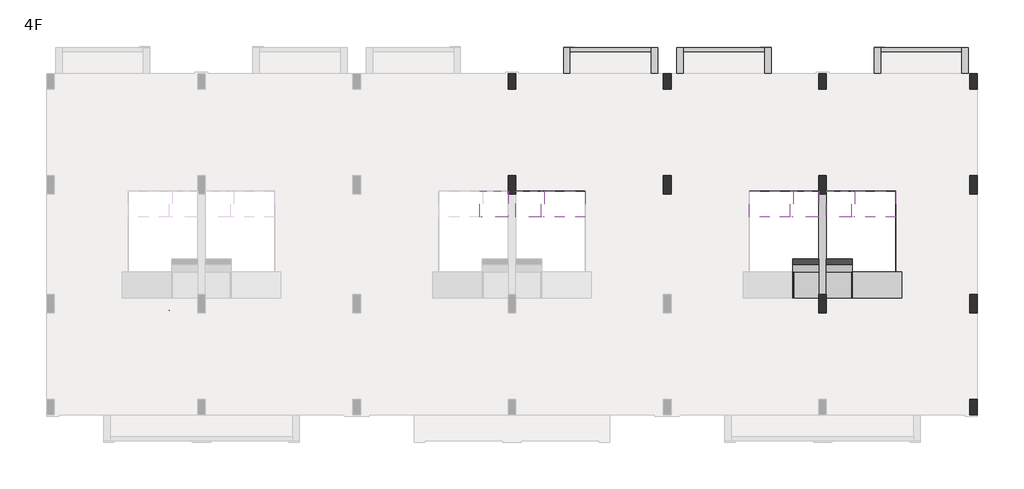
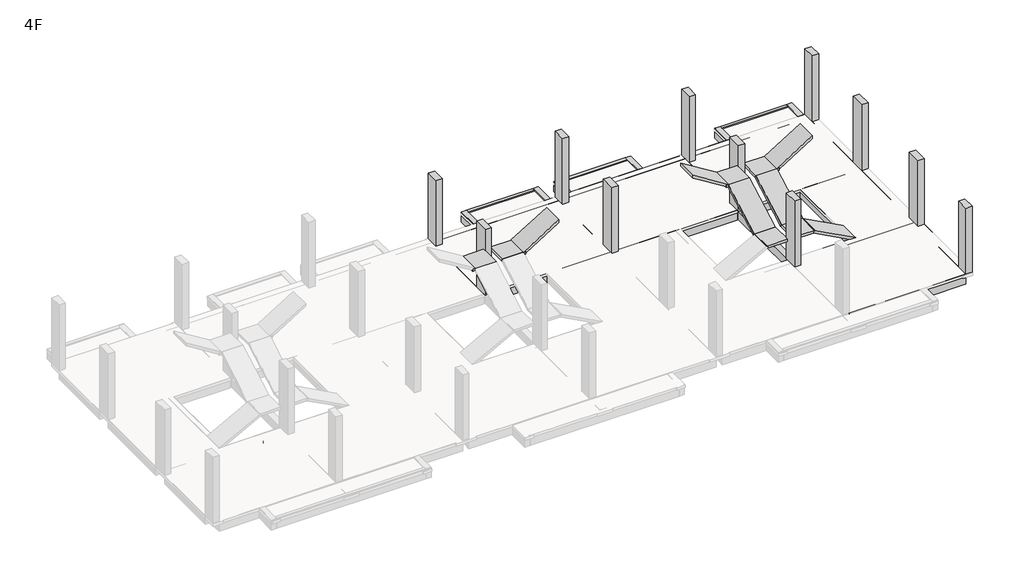
# One storey, part 3 of 3: 37 beams, 11 columns, 1 proxy.
"""IFC4 building model written with IfcOpenShell, lengths in millimetres."""

import ifcopenshell
import ifcopenshell.guid

model = None  # the IFC model being written
_history = None  # IfcOwnerHistory: only IFC2X3 demands one
_inside = {}  # id of a spatial element -> (the spatial element, [elements in it])
_under = {}  # id of a project, library or spatial element -> (it, [spatial elements below it])
_declared = {}  # id of a project -> (the project, [libraries it declares])
_typed = {}  # id of a type object -> (the type object, [elements of that type])
_made_of = {}  # id of a material, layer set ... -> (it, [elements and type objects made of it])


def new_model(schema):
    """Start an empty IFC model of exactly this schema.

    Asked for "IFC4X3", IfcOpenShell would pick the latest addendum, in which some entities
    have other attributes; the version numbers below select the first issue.
    IFC2X3 requires an IfcOwnerHistory on every rooted entity: one is made here for all.
    """
    global model, _history
    if schema == "IFC4X3":
        model = ifcopenshell.file(schema_version=(4, 3, 0, 0))
    else:
        model = ifcopenshell.file(schema=schema)
    _inside.clear()
    _under.clear()
    _declared.clear()
    _typed.clear()
    _made_of.clear()
    _history = None
    if model.schema == "IFC2X3":
        org = make("IfcOrganization", Name="unknown")
        user = make(
            "IfcPersonAndOrganization",
            ThePerson=make("IfcPerson", FamilyName="unknown"),
            TheOrganization=org,
        )
        app = make(
            "IfcApplication",
            ApplicationDeveloper=org,
            Version="unknown",
            ApplicationFullName="unknown",
            ApplicationIdentifier="unknown",
        )
        _history = make(
            "IfcOwnerHistory",
            OwningUser=user,
            OwningApplication=app,
            ChangeAction="ADDED",
            CreationDate=0,
        )
    return model


def make(cls, **values):
    """One entity of the class cls with the attributes given. An attribute that is None is left unset."""
    return model.create_entity(
        cls, **{name: value for name, value in values.items() if value is not None}
    )


def rooted(cls, **values):
    """An entity with a GlobalId (a new one), such as an element, a storey or a relation."""
    return make(cls, GlobalId=ifcopenshell.guid.new(), OwnerHistory=_history, **values)


def si_unit(unit_type, name, prefix=None):
    """IfcSIUnit, for example si_unit("LENGTHUNIT", "METRE", prefix="MILLI")."""
    return make("IfcSIUnit", UnitType=unit_type, Prefix=prefix, Name=name)


def assignment(units):
    """IfcUnitAssignment: the units of a project."""
    return None if units is None else make("IfcUnitAssignment", Units=units)


def point(xyz):
    """IfcCartesianPoint."""
    return None if xyz is None else make("IfcCartesianPoint", Coordinates=xyz)


def direction(xyz):
    """IfcDirection."""
    return None if xyz is None else make("IfcDirection", DirectionRatios=xyz)


def frame(location, z_axis=None, x_axis=None):
    """IfcAxis2Placement3D, a coordinate frame: its origin and axes. An axis left out is left unset."""
    return make(
        "IfcAxis2Placement3D",
        Location=point(location),
        Axis=direction(z_axis),
        RefDirection=direction(x_axis),
    )


def frame_2d(location, x_axis=None):
    """IfcAxis2Placement2D, a coordinate frame in the plane: its origin and x axis."""
    return make(
        "IfcAxis2Placement2D", Location=point(location), RefDirection=direction(x_axis)
    )


def origin():
    """The frame at (0, 0, 0) with its axes left unset."""
    return frame((0.0, 0.0, 0.0))


def origin_with_axes():
    """The frame at (0, 0, 0) with the z axis (0, 0, 1) and the x axis (1, 0, 0) written out."""
    return frame((0.0, 0.0, 0.0), z_axis=(0.0, 0.0, 1.0), x_axis=(1.0, 0.0, 0.0))


def place(relative_to, where):
    """IfcLocalPlacement: puts the frame where relative to a parent placement (None: the world)."""
    return make(
        "IfcLocalPlacement", PlacementRelTo=relative_to, RelativePlacement=where
    )


def context(
    kind, dimensions, precision=None, world=None, true_north=None, identifier=None
):
    """IfcGeometricRepresentationContext, for example the 3D "Model" context."""
    return make(
        "IfcGeometricRepresentationContext",
        ContextIdentifier=identifier,
        ContextType=kind,
        CoordinateSpaceDimension=dimensions,
        Precision=precision,
        WorldCoordinateSystem=world,
        TrueNorth=true_north,
    )


def project(units=None, contexts=None):
    """IfcProject with its units and contexts."""
    return rooted(
        "IfcProject",
        Name="project",
        RepresentationContexts=contexts,
        UnitsInContext=assignment(units),
    )


def spatial(cls, under=None, at=None, **own):
    """A site, building, storey or space (cls), placed at a placement, below another one or the project."""
    s = rooted(cls, ObjectPlacement=at, **own)
    if under is not None:
        _under.setdefault(under.id(), (under, []))[1].append(s)
    return s


def polyline(points):
    """IfcPolyline through the points."""
    return make("IfcPolyline", Points=[point(p) for p in points])


def circle_curve(where, radius):
    """IfcCircle in the frame where."""
    return make("IfcCircle", Position=where, Radius=radius)


def ellipse_curve(where, semi_axis1, semi_axis2):
    """IfcEllipse in the frame where."""
    return make(
        "IfcEllipse", Position=where, SemiAxis1=semi_axis1, SemiAxis2=semi_axis2
    )


def trimmed(basis, trim1, trim2, sense, master):
    """IfcTrimmedCurve: the piece of a basis curve between two trims."""
    return make(
        "IfcTrimmedCurve",
        BasisCurve=basis,
        Trim1=trim1,
        Trim2=trim2,
        SenseAgreement=sense,
        MasterRepresentation=master,
    )


def segment(curve, same_sense, transition):
    """IfcCompositeCurveSegment."""
    return make(
        "IfcCompositeCurveSegment",
        Transition=transition,
        SameSense=same_sense,
        ParentCurve=curve,
    )


def composite_curve(segments, self_intersect=None):
    """IfcCompositeCurve: segments joined end to end."""
    return make("IfcCompositeCurve", Segments=segments, SelfIntersect=self_intersect)


def outline(outer, holes=None, kind="AREA"):
    """IfcArbitraryClosedProfileDef: a profile drawn as a closed curve; with holes, ...WithVoids."""
    if holes is None:
        return make("IfcArbitraryClosedProfileDef", ProfileType=kind, OuterCurve=outer)
    return make(
        "IfcArbitraryProfileDefWithVoids",
        ProfileType=kind,
        OuterCurve=outer,
        InnerCurves=holes,
    )


def extrude(swept, where, along, depth):
    """IfcExtrudedAreaSolid: the profile swept, set in the frame where, extruded along a direction by depth."""
    return make(
        "IfcExtrudedAreaSolid",
        SweptArea=swept,
        Position=where,
        ExtrudedDirection=direction(along),
        Depth=depth,
    )


def faces_of(points, faces, orient=None, outer=None):
    """IfcFace entities. A face is a list of loops; a loop is a list of indices into points, from 0.

    orient and outer hold one flag for each loop. By default every Orientation is true, the
    first loop of a face is its IfcFaceOuterBound and the others are IfcFaceBound.
    """
    made = []
    for i, loops in enumerate(faces):
        bounds = []
        for j, loop in enumerate(loops):
            is_outer = j == 0 if outer is None else outer[i][j]
            bounds.append(
                make(
                    "IfcFaceOuterBound" if is_outer else "IfcFaceBound",
                    Bound=make("IfcPolyLoop", Polygon=[points[k] for k in loop]),
                    Orientation=True if orient is None else orient[i][j],
                )
            )
        made.append(make("IfcFace", Bounds=bounds))
    return made


def faceted_brep(points, faces, orient=None, outer=None, voids=None):
    """IfcFacetedBrep: a solid bounded by flat faces; with voids (closed shells), ...WithVoids."""
    shared = [point(p) for p in points]
    hull = make("IfcClosedShell", CfsFaces=faces_of(shared, faces, orient, outer))
    if voids is None:
        return make("IfcFacetedBrep", Outer=hull)
    return make(
        "IfcFacetedBrepWithVoids",
        Outer=hull,
        Voids=[
            make(cls, CfsFaces=faces_of(shared, fs, o, b)) for cls, fs, o, b in voids
        ],
    )


def shape(context_of_items, identifier, shape_type, items):
    """IfcShapeRepresentation: the items that make up one representation, for example the "Body"."""
    return make(
        "IfcShapeRepresentation",
        ContextOfItems=context_of_items,
        RepresentationIdentifier=identifier,
        RepresentationType=shape_type,
        Items=items,
    )


def source(mapping_origin, context_of_items, identifier, shape_type, items):
    """IfcRepresentationMap: a shape defined once, which mapped items show again and again."""
    return make(
        "IfcRepresentationMap",
        MappingOrigin=mapping_origin,
        MappedRepresentation=shape(context_of_items, identifier, shape_type, items),
    )


def transform(
    local_origin,
    x_axis=None,
    y_axis=None,
    z_axis=None,
    scale=None,
    scale2=None,
    scale3=None,
    uniform=True,
):
    """IfcCartesianTransformationOperator3D, or its non-uniform kind. x_axis, y_axis, z_axis: its Axis1, 2, 3."""
    if uniform:
        return make(
            "IfcCartesianTransformationOperator3D",
            Axis1=direction(x_axis),
            Axis2=direction(y_axis),
            LocalOrigin=point(local_origin),
            Scale=scale,
            Axis3=direction(z_axis),
        )
    return make(
        "IfcCartesianTransformationOperator3DnonUniform",
        Axis1=direction(x_axis),
        Axis2=direction(y_axis),
        LocalOrigin=point(local_origin),
        Scale=scale,
        Axis3=direction(z_axis),
        Scale2=scale2,
        Scale3=scale3,
    )


def mapped(mapping_source, mapping_target):
    """IfcMappedItem: shows the shape of a source again, moved by a transform."""
    return make(
        "IfcMappedItem", MappingSource=mapping_source, MappingTarget=mapping_target
    )


def made_of(thing, what):
    """Note that an element or type object is made of a material, layer set ...; save() writes the relation."""
    if what is not None:
        _made_of.setdefault(what.id(), (what, []))[1].append(thing)
    return thing


def element(
    cls,
    number,
    at=None,
    inside=None,
    cuts=None,
    type_object=None,
    material=None,
    context=None,
    identifier="Body",
    shape_type=None,
    held_by="IfcProductDefinitionShape",
    body=None,
    shapes=None,
    **own,
):
    """One element of the class cls, such as IfcWall. Its Tag is "e" and its number.

    at: its placement. inside: the storey or other place that contains it. cuts: it is an
    opening in that element (IfcRelVoidsElement). A single representation is given by context,
    identifier, shape_type and body (its items); several are given by shapes. held_by: the class
    of the entity that holds the representations. save() writes the other relations.
    """
    e = rooted(cls, Tag="e%d" % number, ObjectPlacement=at, **own)
    if body is not None:
        shapes = [shape(context, identifier, shape_type, body)]
    if shapes is not None:
        e.Representation = make(held_by, Representations=shapes)
    if inside is not None:
        _inside.setdefault(inside.id(), (inside, []))[1].append(e)
    if cuts is not None:
        rooted(
            "IfcRelVoidsElement", RelatingBuildingElement=cuts, RelatedOpeningElement=e
        )
    if type_object is not None:
        _typed.setdefault(type_object.id(), (type_object, []))[1].append(e)
    return made_of(e, material)


def aggregate(whole, parts):
    """IfcRelAggregates: a whole, such as a stair, and the parts it consists of."""
    return rooted("IfcRelAggregates", RelatingObject=whole, RelatedObjects=parts)


def save(model, path):
    """Write the relations noted so far, then the file.

    IfcRelAggregates (storeys below a building ...), IfcRelContainedInSpatialStructure (elements
    in a storey), IfcRelDefinesByType, IfcRelAssociatesMaterial and IfcRelDeclares: one each for
    every whole, place, type object, material and project.
    """
    for whole, parts in _under.values():
        aggregate(whole, parts)
    for where, things in _inside.values():
        rooted(
            "IfcRelContainedInSpatialStructure",
            RelatedElements=things,
            RelatingStructure=where,
        )
    for kind, things in _typed.values():
        rooted("IfcRelDefinesByType", RelatedObjects=things, RelatingType=kind)
    for what, things in _made_of.values():
        rooted("IfcRelAssociatesMaterial", RelatedObjects=things, RelatingMaterial=what)
    for by, libraries in _declared.values():
        rooted("IfcRelDeclares", RelatingContext=by, RelatedDefinitions=libraries)
    model.write(path)


def plane_surface(at):
    """IfcPlane: the flat surface through the origin of the frame at, square to its z axis."""
    return make("IfcPlane", Position=at)


def cylinder_surface(at, radius):
    """IfcCylindricalSurface: all points at the distance radius from the z axis of the frame at."""
    return make("IfcCylindricalSurface", Position=at, Radius=radius)


def revolved_surface(curve, axis_point, axis_direction):
    """IfcSurfaceOfRevolution: the curve turned about the line through axis_point along axis_direction."""
    return make(
        "IfcSurfaceOfRevolution",
        SweptCurve=make("IfcArbitraryOpenProfileDef", ProfileType="CURVE", Curve=curve),
        AxisPosition=make("IfcAxis1Placement", Location=point(axis_point), Axis=direction(axis_direction)),
    )


def advanced_brep(points, edges, surfaces, faces):
    """IfcAdvancedBrep: a solid bounded by faces that lie on surfaces and meet in shared edges.

    An edge is (start, end): straight between two places in points (the first is 0);
    or (start, end, curve); or (start, end, curve, False) where it runs against its curve.
    A face is (place in surfaces, loops), or (place, loops, False) where it looks against
    its surface's normal. A loop lists edges by number (the first is 1), with a minus sign
    where the edge is run from its end to its start. The first loop is the outer one.
    """
    corners = [point(p) for p in points]
    vertices = [make("IfcVertexPoint", VertexGeometry=c) for c in corners]
    made = []
    for start, end, *more in edges:
        made.append(
            make(
                "IfcEdgeCurve",
                EdgeStart=vertices[start],
                EdgeEnd=vertices[end],
                EdgeGeometry=more[0] if more else make("IfcPolyline", Points=[corners[start], corners[end]]),
                SameSense=more[1] if len(more) > 1 else True,
            )
        )
    hull = []
    for where, loops, *sense in faces:
        bounds = []
        for j, loop in enumerate(loops):
            ring = [make("IfcOrientedEdge", EdgeElement=made[abs(k) - 1], Orientation=k > 0) for k in loop]
            bounds.append(
                make(
                    "IfcFaceOuterBound" if j == 0 else "IfcFaceBound",
                    Bound=make("IfcEdgeLoop", EdgeList=ring),
                    Orientation=True,
                )
            )
        hull.append(make("IfcAdvancedFace", Bounds=bounds, FaceSurface=surfaces[where], SameSense=sense[0] if sense else True))
    return make("IfcAdvancedBrep", Outer=make("IfcClosedShell", CfsFaces=hull))


def m_support_metal_circular_m_support_metal_circular_a779fbb7(model_context):
    return source(origin(), model_context, "Body", "SolidModel", [
        advanced_brep(
        [(-6.0, 0.0, 0.0), (6.0, 0.0, 0.0), (-6.0, 0.0, -63.0), (6.0, 0.0, -63.0), (6.0, 12.0, -75.0), (-6.0, 12.0, -75.0), (-6.0, 63.0, -75.0), (6.0, 63.0, -75.0)],
        [
            (0, 1, circle_curve(origin_with_axes(), 6.0)),
            (1, 0, circle_curve(origin_with_axes(), 6.0)),
            (0, 2),
            (2, 3, circle_curve(frame((0.0, 0.0, -63.0), z_axis=(0.0, 0.0, 1.0), x_axis=(1.0, 0.0, 0.0)), 6.0)),
            (3, 1),
            (3, 2, circle_curve(frame((0.0, 0.0, -63.0), z_axis=(0.0, 0.0, 1.0), x_axis=(1.0, 0.0, 0.0)), 6.0)),
            (4, 3, circle_curve(frame((6.0, 12.0, -63.0), z_axis=(-1.0, 0.0, 0.0), x_axis=(0.0, -1.0, 0.0)), 12.0)),
            (2, 5, circle_curve(frame((-6.0, 12.0, -63.0), z_axis=(1.0, 0.0, 0.0), x_axis=(0.0, -1.0, 0.0)), 12.0)),
            (5, 4, circle_curve(frame((0.0, 12.0, -75.0), z_axis=(0.0, -1.0, 0.0), x_axis=(1.0, 0.0, 0.0)), 6.0)),
            (4, 5, circle_curve(frame((0.0, 12.0, -75.0), z_axis=(0.0, -1.0, 0.0), x_axis=(1.0, 0.0, 0.0)), 6.0)),
            (6, 7, circle_curve(frame((0.0, 63.0, -75.0), z_axis=(0.0, 1.0, 0.0), x_axis=(1.0, 0.0, 0.0)), 6.0)),
            (7, 6, circle_curve(frame((0.0, 63.0, -75.0), z_axis=(0.0, 1.0, 0.0), x_axis=(1.0, 0.0, 0.0)), 6.0)),
            (5, 6),
            (7, 4),
        ],
        [
            plane_surface(origin_with_axes()),
            cylinder_surface(origin_with_axes(), 6.0),
            revolved_surface(trimmed(ellipse_curve(frame((0.0, 0.0, -63.0), z_axis=(0.0, 0.0, 1.0), x_axis=(1.0, 0.0, 0.0)), 6.0, 6.0), [point((-6.0, 0.0, -63.0))], [point((6.0, 0.0, -63.0))], True, "CARTESIAN"), (0.0, 12.0, -63.0), (1.0, 0.0, 0.0)),
            revolved_surface(trimmed(ellipse_curve(frame((0.0, 0.0, -63.0), z_axis=(0.0, 0.0, 1.0), x_axis=(1.0, 0.0, 0.0)), 6.0, 6.0), [point((6.0, 0.0, -63.0))], [point((-6.0, 0.0, -63.0))], True, "CARTESIAN"), (0.0, 12.0, -63.0), (1.0, 0.0, 0.0)),
            plane_surface(frame((0.0, 63.0, -75.0), z_axis=(0.0, 1.0, 0.0), x_axis=(1.0, 0.0, 0.0))),
            cylinder_surface(frame((0.0, 12.0, -75.0), z_axis=(0.0, -1.0, 0.0), x_axis=(1.0, 0.0, 0.0)), 6.0),
        ],
        [
            (0, [[1, 2]]),
            (1, [[-1, 3, 4, 5]]),
            (1, [[-2, -5, 6, -3]]),
            (2, [[7, -4, 8, 9]]),
            (3, [[-8, -6, -7, 10]]),
            (4, [[11, 12]]),
            (5, [[-9, 13, -12, 14]]),
            (5, [[-10, -14, -11, -13]]),
        ],
    ),
        extrude(outline(composite_curve([segment(trimmed(circle_curve(frame_2d((-75.0, 0.0)), 25.0), [point((-75.0, -25.0))], [point((-75.0, 25.0))], False, "CARTESIAN"), True, "CONTINUOUS"), segment(trimmed(circle_curve(frame_2d((-75.0, 0.0)), 25.0), [point((-75.0, 25.0))], [point((-75.0, -25.0))], False, "CARTESIAN"), True, "CONTINUOUS")], self_intersect=False)), frame((0.0, 63.0, 0.0), z_axis=(0.0, 1.0, 0.0), x_axis=(0.0, 0.0, 1.0)), (0.0, 0.0, 1.0), 12.0),
    ])


model = new_model("IFC4")

# Units and contexts
model_context = context("Model", 3, world=origin())
ifc_project = project(units=[si_unit("LENGTHUNIT", "METRE", prefix="MILLI")], contexts=[model_context])

# Site, building, storey
site = spatial("IfcSite", under=ifc_project)
building = spatial("IfcBuilding", under=site)
storey = spatial("IfcBuildingStorey", under=building, Name="4F", Elevation=10630.0)

# Beams
placement = place(None, origin())
element("IfcBeam", 1, ObjectType="M_Concrete-Rectangular Beam : 1000x120", at=placement, inside=storey, context=model_context, shape_type="Brep", body=[
    faceted_brep([(16600.0000058, 7550.0000002, 12880.0), (16600.0000058, 8550.0000002, 12880.0), (16600.0000058, 8550.0000002, 12760.0), (16600.0000058, 7550.0000002, 12760.0), (17700.0000058, 8550.0000002, 12760.0), (17700.0000058, 8550.0000002, 12880.0), (17700.0000058, 7550.0000002, 12880.0), (17700.0000058, 7609.0063595, 12775.5095719), (17700.0000058, 7581.5414925, 12760.0), (16700.0000058, 7550.0000002, 12880.0), (16700.0000058, 7581.5414925, 12760.0), (16700.0000058, 7550.0000002, 12760.0), (16700.0000058, 7609.0063595, 12775.5095719)], [[[0, 1, 2, 3]], [[4, 5, 6, 7, 8]], [[1, 0, 9, 6, 5]], [[2, 1, 5, 4]], [[3, 2, 4, 8, 10, 11]], [[0, 3, 11, 9]], [[12, 7, 6, 9]], [[7, 12, 10, 8]], [[12, 9, 11, 10]]]),
])
element("IfcBeam", 2, ObjectType="M_Concrete-Rectangular Beam : 1000x120", at=placement, inside=storey, context=model_context, shape_type="Brep", body=[
    faceted_brep([(19100.0000058, 8550.0000002, 12880.0), (19100.0000058, 7550.0000002, 12880.0), (19100.0000058, 7550.0000002, 12760.0), (19100.0000058, 8550.0000002, 12760.0), (18000.0000058, 8550.0000002, 12880.0), (18000.0000058, 8550.0000002, 12760.0), (18000.0000058, 7581.5414925, 12760.0), (18000.0000058, 7609.0063595, 12775.5095719), (18000.0000058, 7550.0000002, 12880.0), (19000.0000058, 7550.0000002, 12880.0), (19000.0000058, 7550.0000002, 12760.0), (19000.0000058, 7581.5414925, 12760.0), (19000.0000058, 7609.0063595, 12775.5095719)], [[[0, 1, 2, 3]], [[4, 5, 6, 7, 8]], [[1, 0, 4, 8, 9]], [[0, 3, 5, 4]], [[3, 2, 10, 11, 6, 5]], [[2, 1, 9, 10]], [[12, 9, 8, 7]], [[12, 7, 6, 11]], [[9, 12, 11, 10]]]),
])
element("IfcBeam", 3, ObjectType="M_Concrete-Rectangular Beam : 1000x120", at=placement, inside=storey, context=model_context, shape_type="Brep", body=[
    faceted_brep([(18984.2496976, 7549.9999993, 12880.0), (20680.0000464, 7549.9999993, 13930.0), (20680.0000058, 8549.9999993, 13929.9999748), (18984.2496976, 8549.9999993, 12880.0), (20680.0000058, 8549.9999993, 13788.8582241), (19100.0000058, 8549.9999993, 12810.5302519), (19100.0000058, 8549.9999993, 12880.0), (19100.0000058, 7549.9999993, 12810.5302519), (20680.0000058, 7549.9999993, 13788.8582241), (19000.0000058, 7549.9999993, 12880.0), (19100.0000058, 7549.9999993, 12880.0)], [[[0, 1, 2, 3]], [[3, 2, 4, 5, 6]], [[7, 5, 4, 8]], [[1, 0, 9, 10, 7, 8]], [[10, 6, 5, 7]], [[6, 10, 9, 0, 3]], [[2, 1, 8, 4]]]),
])
element("IfcBeam", 4, ObjectType="M_Concrete-Rectangular Beam : 1000x120", at=placement, inside=storey, context=model_context, shape_type="Brep", body=[
    faceted_brep([(28700.0000039, 7550.0000002, 12880.0), (29700.0000039, 7550.0000002, 12880.0), (29700.0000039, 7609.0063595, 12775.5095719), (28700.0000039, 7609.0063595, 12775.5095719), (28700.0000039, 5424.9999998, 11680.0), (28700.0000039, 5484.0063591, 11575.5095719), (29700.0000039, 5484.0063591, 11575.5095719), (29700.0000039, 5424.9999998, 11680.0), (29700.0000039, 5524.9999998, 11598.6589219), (29700.0000039, 7581.5414925, 12760.0), (28700.0000039, 5524.9999998, 11598.6589219), (28700.0000039, 7581.5414925, 12760.0)], [[[0, 1, 2, 3]], [[4, 5, 6, 7]], [[1, 0, 4, 7]], [[2, 1, 7, 6, 8, 9]], [[3, 2, 9, 8, 6, 5, 10, 11]], [[0, 3, 11, 10, 5, 4]]]),
])
element("IfcBeam", 5, ObjectType="M_Concrete-Rectangular Beam : 1000x120", at=placement, inside=storey, context=model_context, shape_type="Brep", body=[
    faceted_brep([(28600.0000039, 7550.0000002, 12880.0), (28600.0000039, 8550.0000002, 12880.0), (28600.0000039, 8550.0000002, 12760.0), (28600.0000039, 7550.0000002, 12760.0), (29700.0000039, 8550.0000002, 12760.0), (29700.0000039, 8550.0000002, 12880.0), (29700.0000039, 7550.0000002, 12880.0), (29700.0000039, 7609.0063595, 12775.5095719), (29700.0000039, 7581.5414925, 12760.0), (28700.0000039, 7550.0000002, 12880.0), (28700.0000039, 7581.5414925, 12760.0), (28700.0000039, 7550.0000002, 12760.0), (28700.0000039, 7609.0063595, 12775.5095719)], [[[0, 1, 2, 3]], [[4, 5, 6, 7, 8]], [[1, 0, 9, 6, 5]], [[2, 1, 5, 4]], [[3, 2, 4, 8, 10, 11]], [[0, 3, 11, 9]], [[12, 7, 6, 9]], [[7, 12, 10, 8]], [[12, 9, 11, 10]]]),
])
element("IfcBeam", 6, ObjectType="M_Concrete-Rectangular Beam : 1000x120", at=placement, inside=storey, context=model_context, shape_type="Brep", body=[
    faceted_brep([(27019.9999632, 7549.9999993, 13930.0), (28715.750312, 7549.9999993, 12880.0), (28715.750312, 8549.9999993, 12880.0), (27019.9999632, 8549.9999993, 13930.0), (28600.0000039, 8549.9999993, 12880.0), (28600.0000039, 8549.9999993, 12810.5302519), (27020.000004, 8549.9999993, 13788.8582239), (28600.0000039, 7549.9999993, 12810.5302519), (27020.000004, 7549.9999993, 13788.8582239), (28600.0000039, 7549.9999993, 12880.0), (28700.0000039, 7549.9999993, 12880.0)], [[[0, 1, 2, 3]], [[3, 2, 4, 5, 6]], [[5, 7, 8, 6]], [[1, 0, 8, 7, 9, 10]], [[4, 9, 7, 5]], [[9, 4, 2, 1, 10]], [[0, 3, 6, 8]]]),
])
element("IfcBeam", 7, ObjectType="M_Concrete-Rectangular Beam : 1000x120", at=placement, inside=storey, context=model_context, shape_type="Brep", body=[
    faceted_brep([(29700.0000039, 5524.9999998, 11560.0), (28700.0000039, 5524.9999998, 11560.0), (28700.0000039, 5524.9999998, 11598.6589219), (29700.0000039, 5524.9999998, 11598.6589219), (29700.0000039, 4424.9999998, 11560.0), (29700.0000039, 4424.9999998, 11680.0), (28730.4772098, 4424.9999998, 11680.0), (28787.1330609, 4424.9999998, 11574.2166623), (28760.5888301, 4424.9999998, 11560.0), (29700.0000039, 5424.9999998, 11680.0), (28700.0000039, 5424.9999998, 11680.0), (28700.0000039, 4424.9999998, 11680.0), (29700.0000039, 5484.0063591, 11575.5095719), (28760.5888301, 5424.9999998, 11560.0), (28700.0000039, 5424.9999998, 11560.0), (28700.0000039, 4424.9999998, 11663.6768996), (28700.0000039, 5484.0063591, 11575.5095719), (28700.0000039, 5424.9999998, 11663.6768996), (28730.4772098, 5424.9999998, 11680.0), (28787.1330609, 5424.9999998, 11574.2166623)], [[[0, 1, 2, 3]], [[4, 5, 6, 7, 8]], [[6, 5, 9, 10, 11]], [[5, 4, 0, 3, 12, 9]], [[1, 0, 4, 8, 13, 14]], [[15, 11, 10, 16, 2, 1, 14, 17]], [[6, 18, 19, 7]], [[18, 6, 15, 17]], [[7, 19, 13, 8]], [[19, 18, 17, 14, 13]], [[11, 15, 6]], [[12, 16, 10, 9]], [[16, 12, 3, 2]]]),
])
element("IfcBeam", 8, ObjectType="M_Concrete-Rectangular Beam : 1000x120", at=placement, inside=storey, context=model_context, shape_type="Brep", body=[
    faceted_brep([(30969.5227979, 4424.9999998, 11680.0), (30969.5227979, 5424.9999998, 11680.0), (30912.8669468, 5424.9999998, 11574.2166623), (30912.8669468, 4424.9999998, 11574.2166623), (31000.0000039, 4424.9999998, 11663.6768996), (32930.0000046, 4424.9999998, 10630.0), (32930.0000046, 5424.9999998, 10630.0), (31000.0000039, 5424.9999998, 11663.6768996), (30939.4111776, 4424.9999998, 11560.0), (32675.8338464, 4424.9999998, 10630.0), (30939.4111776, 5424.9999998, 11560.0), (32680.0000108, 5424.9999998, 10627.7686695), (32680.0000108, 4449.9999998, 10627.7686695), (32675.8338464, 4449.9999998, 10630.0), (32680.0000108, 5424.9999998, 10630.0), (32680.0000108, 4449.9999998, 10630.0)], [[[0, 1, 2, 3]], [[1, 0, 4, 5, 6, 7]], [[0, 3, 8, 9, 5, 4]], [[3, 2, 10, 11, 12, 13, 9, 8]], [[2, 1, 7, 6, 14, 11, 10]], [[9, 13, 15, 14, 6, 5]], [[11, 14, 15, 12]], [[15, 13, 12]]]),
])
element("IfcBeam", 9, ObjectType="M_Concrete-Rectangular Beam : 1000x120", at=placement, inside=storey, context=model_context, shape_type="Brep", body=[
    faceted_brep([(31000.0000039, 7550.0000002, 12880.0), (31000.0000039, 7609.0063595, 12775.5095719), (30000.0000039, 7609.0063595, 12775.5095719), (30000.0000039, 7550.0000002, 12880.0), (31000.0000039, 5424.9999998, 11680.0), (30000.0000039, 5424.9999998, 11680.0), (30000.0000039, 5484.0063591, 11575.5095719), (31000.0000039, 5484.0063591, 11575.5095719), (30000.0000039, 7581.5414925, 12760.0), (30000.0000039, 5524.9999998, 11598.6589219), (31000.0000039, 7581.5414925, 12760.0), (31000.0000039, 5524.9999998, 11598.6589219)], [[[0, 1, 2, 3]], [[4, 5, 6, 7]], [[3, 5, 4, 0]], [[2, 8, 9, 6, 5, 3]], [[1, 10, 11, 7, 6, 9, 8, 2]], [[0, 4, 7, 11, 10, 1]]]),
])
element("IfcBeam", 10, ObjectType="M_Concrete-Rectangular Beam : 1000x120", at=placement, inside=storey, context=model_context, shape_type="Brep", body=[
    faceted_brep([(31100.0000039, 8550.0000002, 12880.0), (31100.0000039, 7550.0000002, 12880.0), (31100.0000039, 7550.0000002, 12760.0), (31100.0000039, 8550.0000002, 12760.0), (30000.0000039, 8550.0000002, 12880.0), (30000.0000039, 8550.0000002, 12760.0), (30000.0000039, 7581.5414925, 12760.0), (30000.0000039, 7609.0063595, 12775.5095719), (30000.0000039, 7550.0000002, 12880.0), (31000.0000039, 7550.0000002, 12880.0), (31000.0000039, 7550.0000002, 12760.0), (31000.0000039, 7581.5414925, 12760.0), (31000.0000039, 7609.0063595, 12775.5095719)], [[[0, 1, 2, 3]], [[4, 5, 6, 7, 8]], [[1, 0, 4, 8, 9]], [[0, 3, 5, 4]], [[3, 2, 10, 11, 6, 5]], [[2, 1, 9, 10]], [[12, 9, 8, 7]], [[12, 7, 6, 11]], [[9, 12, 11, 10]]]),
])
element("IfcBeam", 11, ObjectType="M_Concrete-Rectangular Beam : 1000x120", at=placement, inside=storey, context=model_context, shape_type="Brep", body=[
    faceted_brep([(30984.2496957, 7549.9999993, 12880.0), (32680.0000445, 7549.9999993, 13930.0), (32680.0000108, 8549.9999993, 13929.9999791), (30984.2496957, 8549.9999993, 12880.0), (32680.0000108, 8549.9999993, 13788.8582284), (31100.0000039, 8549.9999993, 12810.5302519), (31100.0000039, 8549.9999993, 12880.0), (31100.0000039, 7549.9999993, 12810.5302519), (32680.0000108, 7549.9999993, 13788.8582284), (31000.0000039, 7549.9999993, 12880.0), (31100.0000039, 7549.9999993, 12880.0)], [[[0, 1, 2, 3]], [[3, 2, 4, 5, 6]], [[7, 5, 4, 8]], [[1, 0, 9, 10, 7, 8]], [[10, 6, 5, 7]], [[6, 10, 9, 0, 3]], [[2, 1, 8, 4]]]),
])
element("IfcBeam", 12, ObjectType="M_Concrete-Rectangular Beam : 1000x120", at=placement, inside=storey, context=model_context, shape_type="Brep", body=[
    faceted_brep([(31000.0000039, 5524.9999998, 11560.0), (30000.0000039, 5524.9999998, 11560.0), (30000.0000039, 5524.9999998, 11598.6589219), (31000.0000039, 5524.9999998, 11598.6589219), (30000.0000039, 4424.9999998, 11680.0), (30000.0000039, 4424.9999998, 11560.0), (30939.4111776, 4424.9999998, 11560.0), (30912.8669468, 4424.9999998, 11574.2166623), (30969.5227979, 4424.9999998, 11680.0), (31000.0000039, 4424.9999998, 11680.0), (31000.0000039, 5424.9999998, 11680.0), (30000.0000039, 5424.9999998, 11680.0), (30000.0000039, 5484.0063591, 11575.5095719), (31000.0000039, 5424.9999998, 11560.0), (30939.4111776, 5424.9999998, 11560.0), (31000.0000039, 4424.9999998, 11663.6768996), (31000.0000039, 5424.9999998, 11663.6768996), (31000.0000039, 5484.0063591, 11575.5095719), (30969.5227979, 5424.9999998, 11680.0), (30912.8669468, 5424.9999998, 11574.2166623)], [[[0, 1, 2, 3]], [[4, 5, 6, 7, 8]], [[8, 9, 10, 11, 4]], [[5, 4, 11, 12, 2, 1]], [[1, 0, 13, 14, 6, 5]], [[9, 15, 16, 13, 0, 3, 17, 10]], [[18, 8, 7, 19]], [[8, 18, 16, 15]], [[19, 7, 6, 14]], [[18, 19, 14, 13, 16]], [[15, 9, 8]], [[17, 12, 11, 10]], [[12, 17, 3, 2]]]),
])
element("IfcBeam", 13, ObjectType="M_Concrete-Rectangular Beam : 150x500", at=placement, inside=storey, context=model_context, shape_type="SweptSolid", body=[
    extrude(outline(polyline([(23225.0000411, 14100.0000002), (23225.0000411, 13950.0000002), (20090.0434261, 13950.0000002), (20090.0434261, 14100.0000002), (23225.0000411, 14100.0000002)])), frame((0.0, 0.0, 10130.0), z_axis=(0.0, 0.0, 1.0), x_axis=(1.0, 0.0, 0.0)), (0.0, 0.0, 1.0), 500.0),
])
element("IfcBeam", 14, ObjectType="M_Concrete-Rectangular Beam : 150x500", at=placement, inside=storey, context=model_context, shape_type="SweptSolid", body=[
    extrude(outline(polyline([(27609.7271083, 14100.0000002), (27609.7271083, 13950.0000002), (24475.0998348, 13950.0000002), (24475.0998348, 14100.0000002), (27609.7271083, 14100.0000002)])), frame((0.0, 0.0, 10130.0), z_axis=(0.0, 0.0, 1.0), x_axis=(1.0, 0.0, 0.0)), (0.0, 0.0, 1.0), 500.0),
])
element("IfcBeam", 15, ObjectType="M_Concrete-Rectangular Beam : 150x500", at=placement, inside=storey, context=model_context, shape_type="SweptSolid", body=[
    extrude(outline(polyline([(35224.9001759, 14100.0000002), (35224.9001759, 13950.0000002), (32090.0000473, 13950.0000002), (32090.0000473, 14100.0000002), (35224.9001759, 14100.0000002)])), frame((0.0, 0.0, 10130.0), z_axis=(0.0, 0.0, 1.0), x_axis=(1.0, 0.0, 0.0)), (0.0, 0.0, 1.0), 500.0),
])
element("IfcBeam", 16, ObjectType="M_Concrete-Rectangular Beam : 250x400", at=placement, inside=storey, context=model_context, shape_type="Brep", body=[
    faceted_brep([(32930.0000108, 8549.9999993, 10630.0), (32680.0000108, 8549.9999993, 10630.0), (32680.0000108, 5424.9999998, 10630.0), (32680.0000108, 4449.9999998, 10630.0), (32930.0000108, 4449.9999998, 10630.0), (32930.0000108, 8549.9999993, 10230.0), (32930.0000108, 4449.9999998, 10230.0), (32680.0000108, 8549.9999993, 10230.0), (32680.0000108, 4449.9999998, 10230.0), (32680.0000108, 8549.9999993, 10488.8582284), (32680.0000108, 4449.9999998, 10627.7686695)], [[[0, 1, 2, 3, 4]], [[5, 0, 4, 6]], [[7, 5, 6, 8]], [[1, 9, 7, 8, 10, 3, 2]], [[1, 0, 5, 7, 9]], [[4, 3, 10, 8, 6]]]),
])
element("IfcBeam", 17, ObjectType="M_Concrete-Rectangular Beam : 250x500", at=placement, inside=storey, context=model_context, shape_type="Brep", body=[
    faceted_brep([(23475.0000411, 14100.0000002, 10630.0), (23225.0000411, 14100.0000002, 10630.0), (23225.0000411, 13950.0000002, 10630.0), (23225.0000411, 13100.0000001, 10630.0), (23475.0000411, 13100.0000001, 10630.0), (23225.0000411, 14100.0000002, 10130.0), (23225.0000411, 13950.0000002, 10130.0), (23225.0000411, 13100.0000001, 10130.0), (23475.0000411, 14100.0000002, 10130.0), (23475.0000411, 13100.0000001, 10130.0)], [[[0, 1, 2, 3, 4]], [[1, 5, 6, 7, 3, 2]], [[5, 8, 9, 7, 6]], [[8, 0, 4, 9]], [[1, 0, 8, 5]], [[4, 3, 7, 9]]]),
])
element("IfcBeam", 18, ObjectType="M_Concrete-Rectangular Beam : 250x500", at=placement, inside=storey, context=model_context, shape_type="Brep", body=[
    faceted_brep([(20090.0434261, 14100.0000002, 10630.0), (19840.0434261, 14100.0000002, 10630.0), (19840.0434261, 13100.0000001, 10630.0), (20090.0434261, 13100.0000001, 10630.0), (20090.0434261, 13950.0000002, 10630.0), (19840.0434261, 14100.0000002, 10130.0), (19840.0434261, 13100.0000001, 10130.0), (20090.0434261, 14100.0000002, 10130.0), (20090.0434261, 13950.0000002, 10130.0), (20090.0434261, 13100.0000001, 10130.0)], [[[0, 1, 2, 3, 4]], [[1, 5, 6, 2]], [[5, 7, 8, 9, 6]], [[7, 0, 4, 3, 9, 8]], [[1, 0, 7, 5]], [[3, 2, 6, 9]]]),
])
element("IfcBeam", 19, ObjectType="M_Concrete-Rectangular Beam : 250x500", at=placement, inside=storey, context=model_context, shape_type="Brep", body=[
    faceted_brep([(24475.0998348, 14100.0000002, 10630.0), (24225.0998348, 14100.0000002, 10630.0), (24225.0998348, 13100.0000001, 10630.0), (24475.0998348, 13100.0000001, 10630.0), (24475.0998348, 13950.0000002, 10630.0), (24475.0998348, 14100.0000002, 10130.0), (24475.0998348, 13100.0000001, 10130.0), (24475.0998348, 13950.0000002, 10130.0), (24225.0998348, 14100.0000002, 10130.0), (24225.0998348, 13100.0000001, 10130.0)], [[[0, 1, 2, 3, 4]], [[5, 0, 4, 3, 6, 7]], [[8, 5, 7, 6, 9]], [[1, 8, 9, 2]], [[1, 0, 5, 8]], [[3, 2, 9, 6]]]),
])
element("IfcBeam", 20, ObjectType="M_Concrete-Rectangular Beam : 250x500", at=placement, inside=storey, context=model_context, shape_type="Brep", body=[
    faceted_brep([(27859.7271083, 14100.0000002, 10630.0), (27609.7271083, 14100.0000002, 10630.0), (27609.7271083, 13950.0000002, 10630.0), (27609.7271083, 13100.0000001, 10630.0), (27859.7271083, 13100.0000001, 10630.0), (27859.7271083, 14100.0000002, 10130.0), (27859.7271083, 13100.0000001, 10130.0), (27609.7271083, 14100.0000002, 10130.0), (27609.7271083, 13100.0000001, 10130.0), (27609.7271083, 13950.0000002, 10130.0)], [[[0, 1, 2, 3, 4]], [[5, 0, 4, 6]], [[7, 5, 6, 8, 9]], [[1, 7, 9, 8, 3, 2]], [[1, 0, 5, 7]], [[4, 3, 8, 6]]]),
])
element("IfcBeam", 21, ObjectType="M_Concrete-Rectangular Beam : 250x500", at=placement, inside=storey, context=model_context, shape_type="Brep", body=[
    faceted_brep([(35474.9001759, 14100.0000002, 10630.0), (35224.9001759, 14100.0000002, 10630.0), (35224.9001759, 13950.0000002, 10630.0), (35224.9001759, 13100.0000001, 10630.0), (35474.9001759, 13100.0000001, 10630.0), (35224.9001759, 14100.0000002, 10130.0), (35224.9001759, 13950.0000002, 10130.0), (35224.9001759, 13100.0000001, 10130.0), (35474.9001759, 14100.0000002, 10130.0), (35474.9001759, 13100.0000001, 10130.0)], [[[0, 1, 2, 3, 4]], [[1, 5, 6, 7, 3, 2]], [[5, 8, 9, 7, 6]], [[8, 0, 4, 9]], [[1, 0, 8, 5]], [[4, 3, 7, 9]]]),
])
element("IfcBeam", 22, ObjectType="M_Concrete-Rectangular Beam : 250x500", at=placement, inside=storey, context=model_context, shape_type="Brep", body=[
    faceted_brep([(32090.0000473, 14100.0000002, 10630.0), (31840.0000473, 14100.0000002, 10630.0), (31840.0000473, 13100.0000001, 10630.0), (32090.0000473, 13100.0000001, 10630.0), (32090.0000473, 13950.0000002, 10630.0), (31840.0000473, 14100.0000002, 10130.0), (31840.0000473, 13100.0000001, 10130.0), (32090.0000473, 14100.0000002, 10130.0), (32090.0000473, 13950.0000002, 10130.0), (32090.0000473, 13100.0000001, 10130.0)], [[[0, 1, 2, 3, 4]], [[1, 5, 6, 2]], [[5, 7, 8, 9, 6]], [[7, 0, 4, 3, 9, 8]], [[1, 0, 7, 5]], [[3, 2, 6, 9]]]),
])
element("IfcBeam", 23, ObjectType="M_Concrete-Rectangular Beam : 300x400", at=placement, inside=storey, context=model_context, shape_type="SweptSolid", body=[
    extrude(outline(polyline([(18000.0000046, 9150.0), (17700.0000046, 9150.0), (17700.0000046, 12500.0000005), (18000.0000046, 12500.0000005), (18000.0000046, 9150.0)])), frame((0.0, 0.0, 10230.0), z_axis=(0.0, 0.0, 1.0), x_axis=(1.0, 0.0, 0.0)), (0.0, 0.0, 1.0), 400.0),
])
element("IfcBeam", 24, ObjectType="M_Concrete-Rectangular Beam : 300x400", at=placement, inside=storey, context=model_context, shape_type="SweptSolid", body=[
    extrude(outline(polyline([(30000.0000031, 9150.0000002), (29700.0000031, 9150.0000002), (29700.0000031, 12500.0000005), (30000.0000031, 12500.0000005), (30000.0000031, 9150.0000002)])), frame((0.0, 0.0, 10230.0), z_axis=(0.0, 0.0, 1.0), x_axis=(1.0, 0.0, 0.0)), (0.0, 0.0, 1.0), 400.0),
])
element("IfcBeam", 25, ObjectType="M_Concrete-Rectangular Beam : 300x400", at=placement, inside=storey, context=model_context, shape_type="SweptSolid", body=[
    extrude(outline(polyline([(30000.0000031, 4550.0000002), (29700.0000031, 4550.0000002), (29700.0000031, 8450.0000002), (30000.0000031, 8450.0000002), (30000.0000031, 4550.0000002)])), frame((0.0, 0.0, 10230.0), z_axis=(0.0, 0.0, 1.0), x_axis=(1.0, 0.0, 0.0)), (0.0, 0.0, 1.0), 400.0),
])
element("IfcBeam", 26, ObjectType="M_Concrete-Rectangular Beam : 300x400", at=placement, inside=storey, context=model_context, shape_type="SweptSolid", body=[
    extrude(outline(polyline([(35835.035019, 9150.0000002), (35535.035019, 9150.0000002), (35535.035019, 12500.0000005), (35835.035019, 12500.0000005), (35835.035019, 9150.0000002)])), frame((0.0, 0.0, 10230.0), z_axis=(0.0, 0.0, 1.0), x_axis=(1.0, 0.0, 0.0)), (0.0, 0.0, 1.0), 400.0),
])
element("IfcBeam", 27, ObjectType="M_Concrete-Rectangular Beam : 300x400", at=placement, inside=storey, context=model_context, shape_type="SweptSolid", body=[
    extrude(outline(polyline([(35835.035019, 4550.0000002), (35535.035019, 4550.0000002), (35535.035019, 8450.0000002), (35835.035019, 8450.0000002), (35835.035019, 4550.0000002)])), frame((0.0, 0.0, 10230.0), z_axis=(0.0, 0.0, 1.0), x_axis=(1.0, 0.0, 0.0)), (0.0, 0.0, 1.0), 400.0),
])
element("IfcBeam", 28, ObjectType="M_Concrete-Rectangular Beam : 300x400", at=placement, inside=storey, context=model_context, shape_type="SweptSolid", body=[
    extrude(outline(polyline([(35835.035019, 500.0), (35535.035019, 500.0), (35535.035019, 3850.0000002), (35835.035019, 3850.0000002), (35835.035019, 500.0)])), frame((0.0, 0.0, 10230.0), z_axis=(0.0, 0.0, 1.0), x_axis=(1.0, 0.0, 0.0)), (0.0, 0.0, 1.0), 400.0),
])
element("IfcBeam", 29, ObjectType="M_Concrete-Rectangular Beam : 300x400", at=placement, inside=storey, context=model_context, shape_type="SweptSolid", body=[
    extrude(outline(polyline([(24000.000004, 9150.0000002), (23700.000004, 9150.0000002), (23700.000004, 12500.0000005), (24000.000004, 12500.0000005), (24000.000004, 9150.0000002)])), frame((0.0, 0.0, 10230.0), z_axis=(0.0, 0.0, 1.0), x_axis=(1.0, 0.0, 0.0)), (0.0, 0.0, 1.0), 400.0),
])
element("IfcBeam", 30, ObjectType="M_Concrete-Rectangular Beam : 300x500", at=placement, inside=storey, context=model_context, shape_type="Brep", body=[
    faceted_brep([(18000.0000058, 13100.0000001, 10630.0), (18000.0000058, 12800.0000001, 10630.0), (23700.0000047, 12800.0000001, 10630.0), (23700.0000047, 13100.0000001, 10630.0), (23475.0000411, 13100.0000001, 10630.0), (23225.0000411, 13100.0000001, 10630.0), (20090.0434261, 13100.0000001, 10630.0), (19840.0434261, 13100.0000001, 10630.0), (18000.0000058, 12800.0000001, 10130.0), (23700.0000047, 12800.0000001, 10130.0), (18000.0000058, 13100.0000001, 10130.0), (19840.0434261, 13100.0000001, 10130.0), (20090.0434261, 13100.0000001, 10130.0), (23225.0000411, 13100.0000001, 10130.0), (23475.0000411, 13100.0000001, 10130.0), (23700.0000047, 13100.0000001, 10130.0)], [[[0, 1, 2, 3, 4, 5, 6, 7]], [[1, 8, 9, 2]], [[8, 10, 11, 12, 13, 14, 15, 9]], [[10, 0, 7, 6, 5, 4, 3, 15, 14, 13, 12, 11]], [[1, 0, 10, 8]], [[3, 2, 9, 15]]]),
])
element("IfcBeam", 31, ObjectType="M_Concrete-Rectangular Beam : 300x500", at=placement, inside=storey, context=model_context, shape_type="Brep", body=[
    faceted_brep([(17999.9649983, 8849.9999993, 10630.0), (17999.9649983, 8549.9999993, 10630.0), (20680.0000058, 8549.9999993, 10630.0), (20930.0000058, 8549.9999993, 10630.0), (23699.9649972, 8549.9999993, 10630.0), (23699.9649972, 8849.9999993, 10630.0), (17999.9649983, 8549.9999993, 10130.0), (23699.9649972, 8549.9999993, 10130.0), (17999.9649983, 8849.9999993, 10130.0), (23699.9649972, 8849.9999993, 10130.0)], [[[0, 1, 2, 3, 4, 5]], [[1, 6, 7, 4, 3, 2]], [[6, 8, 9, 7]], [[8, 0, 5, 9]], [[1, 0, 8, 6]], [[5, 4, 7, 9]]]),
])
element("IfcBeam", 32, ObjectType="M_Concrete-Rectangular Beam : 300x500", at=placement, inside=storey, context=model_context, shape_type="Brep", body=[
    faceted_brep([(24000.0000047, 13100.0000001, 10630.0), (24000.000004, 12800.0000001, 10630.0), (29700.0000039, 12800.0000001, 10630.0), (29700.0000039, 13100.0000001, 10630.0), (27859.7271083, 13100.0000001, 10630.0), (27609.7271083, 13100.0000001, 10630.0), (24475.0998348, 13100.0000001, 10630.0), (24225.0998348, 13100.0000001, 10630.0), (24000.0000047, 12800.0000001, 10130.0), (29700.0000039, 12800.0000001, 10130.0), (24000.0000047, 13100.0000001, 10130.0), (24225.0998348, 13100.0000001, 10130.0), (24475.0998348, 13100.0000001, 10130.0), (27609.7271083, 13100.0000001, 10130.0), (27859.7271083, 13100.0000001, 10130.0), (29700.0000039, 13100.0000001, 10130.0)], [[[0, 1, 2, 3, 4, 5, 6, 7]], [[1, 8, 9, 2]], [[8, 10, 11, 12, 13, 14, 15, 9]], [[10, 0, 7, 6, 5, 4, 3, 15, 14, 13, 12, 11]], [[10, 8, 1, 0]], [[3, 2, 9, 15]]]),
])
element("IfcBeam", 33, ObjectType="M_Concrete-Rectangular Beam : 300x500", at=placement, inside=storey, context=model_context, shape_type="Brep", body=[
    faceted_brep([(23999.9649972, 8849.9999993, 10630.0), (23999.9649972, 8549.9999993, 10630.0), (26770.000004, 8549.9999993, 10630.0), (27020.000004, 8549.9999993, 10630.0), (29699.9649964, 8549.9999993, 10630.0), (29699.9649964, 8849.9999993, 10630.0), (23999.9649972, 8549.9999993, 10130.0), (29699.9649964, 8549.9999993, 10130.0), (23999.9649972, 8849.9999993, 10130.0), (29699.9649964, 8849.9999993, 10130.0)], [[[0, 1, 2, 3, 4, 5]], [[1, 6, 7, 4, 3, 2]], [[6, 8, 9, 7]], [[8, 0, 5, 9]], [[1, 0, 8, 6]], [[5, 4, 7, 9]]]),
])
element("IfcBeam", 34, ObjectType="M_Concrete-Rectangular Beam : 300x500", at=placement, inside=storey, context=model_context, shape_type="Brep", body=[
    faceted_brep([(30000.0000039, 13100.0000001, 10630.0), (30000.0000039, 12800.0000001, 10630.0), (35535.035019, 12800.0000001, 10630.0), (35535.035019, 13100.0000001, 10630.0), (35474.9001759, 13100.0000001, 10630.0), (35224.9001759, 13100.0000001, 10630.0), (32090.0000473, 13100.0000001, 10630.0), (31840.0000473, 13100.0000001, 10630.0), (30000.0000039, 12800.0000001, 10130.0), (35535.035019, 12800.0000001, 10130.0), (30000.0000039, 13100.0000001, 10130.0), (31840.0000473, 13100.0000001, 10130.0), (32090.0000473, 13100.0000001, 10130.0), (35224.9001759, 13100.0000001, 10130.0), (35474.9001759, 13100.0000001, 10130.0), (35535.035019, 13100.0000001, 10130.0)], [[[0, 1, 2, 3, 4, 5, 6, 7]], [[1, 8, 9, 2]], [[8, 10, 11, 12, 13, 14, 15, 9]], [[10, 0, 7, 6, 5, 4, 3, 15, 14, 13, 12, 11]], [[1, 0, 10, 8]], [[3, 2, 9, 15]]]),
])
element("IfcBeam", 35, ObjectType="M_Concrete-Rectangular Beam : 300x500", at=placement, inside=storey, context=model_context, shape_type="Brep", body=[
    faceted_brep([(29999.9649964, 8849.9999993, 10630.0), (29999.9649964, 8549.9999993, 10630.0), (32680.0000108, 8549.9999993, 10630.0), (32930.0000108, 8549.9999993, 10630.0), (35535.0000115, 8549.9999993, 10630.0), (35535.0000115, 8849.9999993, 10630.0), (29999.9649964, 8549.9999993, 10130.0), (35535.0000115, 8549.9999993, 10130.0), (29999.9649964, 8849.9999993, 10130.0), (35535.0000115, 8849.9999993, 10130.0)], [[[0, 1, 2, 3, 4, 5]], [[1, 6, 7, 4, 3, 2]], [[6, 8, 9, 7]], [[8, 0, 5, 9]], [[1, 0, 8, 6]], [[5, 4, 7, 9]]]),
])
element("IfcBeam", 36, ObjectType="M_Concrete-Rectangular Beam : 300x500", at=placement, inside=storey, context=model_context, shape_type="Brep", body=[
    faceted_brep([(30000.0000031, 4449.9999998, 10630.0), (30000.0000031, 4149.9999998, 10630.0), (35535.035019, 4149.9999998, 10630.0), (35535.035019, 4449.9999998, 10630.0), (32930.0000108, 4449.9999998, 10630.0), (32680.0000108, 4449.9999998, 10630.0), (32675.8338464, 4449.9999998, 10630.0), (30000.0000039, 4149.9999998, 10130.0), (35535.035019, 4149.9999998, 10130.0), (30000.0000039, 4449.9999998, 10130.0), (35535.035019, 4449.9999998, 10130.0)], [[[0, 1, 2, 3, 4, 5, 6]], [[1, 7, 8, 2]], [[7, 9, 10, 8]], [[9, 0, 6, 5, 4, 3, 10]], [[1, 0, 9, 7]], [[3, 2, 8, 10]]]),
])
element("IfcBeam", 37, ObjectType="M_Concrete-Rectangular Beam : 300x500", at=placement, inside=storey, context=model_context, shape_type="Brep", body=[
    faceted_brep([(30000.0000039, 199.9999987, 10630.0), (30000.0000039, -100.0000013, 10630.0), (33380.0128581, -100.0000013, 10630.0), (33630.0128581, -100.0000013, 10630.0), (35535.035019, -100.0000013, 10630.0), (35535.035019, 199.9999987, 10630.0), (30000.0000039, -100.0000013, 10130.0), (33380.0128581, -100.0000013, 10130.0), (33630.0128581, -100.0000013, 10130.0), (35535.035019, -100.0000013, 10130.0), (30000.0000039, 199.9999987, 10130.0), (35535.035019, 199.9999987, 10130.0)], [[[0, 1, 2, 3, 4, 5]], [[1, 6, 7, 8, 9, 4, 3, 2]], [[6, 10, 11, 9, 8, 7]], [[10, 0, 5, 11]], [[1, 0, 10, 6]], [[5, 4, 9, 11]]]),
])

# Proxy
m_support_metal_circular_m_support_metal_circular_shape = m_support_metal_circular_m_support_metal_circular_a779fbb7(model_context)
element("IfcBuildingElementProxy", 38, Name="M_Support - Metal - Circular : M_Support - Metal - Circular", ObjectType="M_Support - Metal - Circular : M_Support - Metal - Circular", at=placement, inside=storey, context=model_context, shape_type="MappedRepresentation", body=[
    mapped(m_support_metal_circular_m_support_metal_circular_shape, transform((4604.999959, 3949.9999996, 10630.0), x_axis=(1.0, 0.0, 0.0), y_axis=(0.0, 1.0, 0.0), z_axis=(0.0, 0.0, 1.0))),
])

# Columns
element("IfcColumn", 39, ObjectType="M_Concrete-Rectangular-Column : 300x600", at=placement, inside=storey, context=model_context, shape_type="SweptSolid", body=[
    extrude(outline(polyline([(18000.0000058, 13100.0000005), (18000.0000058, 12500.0000005), (17700.0000058, 12500.0000005), (17700.0000058, 13100.0000005), (18000.0000058, 13100.0000005)])), frame((0.0, 0.0, 10630.0), z_axis=(0.0, 0.0, 1.0), x_axis=(1.0, 0.0, 0.0)), (0.0, 0.0, 1.0), 3300.0),
])
element("IfcColumn", 40, ObjectType="M_Concrete-Rectangular-Column : 300x600", at=placement, inside=storey, context=model_context, shape_type="SweptSolid", body=[
    extrude(outline(polyline([(24000.0000047, 13100.0000005), (24000.0000047, 12500.0000005), (23700.0000047, 12500.0000005), (23700.0000047, 13100.0000005), (24000.0000047, 13100.0000005)])), frame((0.0, 0.0, 10630.0), z_axis=(0.0, 0.0, 1.0), x_axis=(1.0, 0.0, 0.0)), (0.0, 0.0, 1.0), 3300.0),
])
element("IfcColumn", 41, ObjectType="M_Concrete-Rectangular-Column : 300x600", at=placement, inside=storey, context=model_context, shape_type="SweptSolid", body=[
    extrude(outline(polyline([(30000.0000039, 13100.0000005), (30000.0000039, 12500.0000005), (29700.0000039, 12500.0000005), (29700.0000039, 13100.0000005), (30000.0000039, 13100.0000005)])), frame((0.0, 0.0, 10630.0), z_axis=(0.0, 0.0, 1.0), x_axis=(1.0, 0.0, 0.0)), (0.0, 0.0, 1.0), 3300.0),
])
element("IfcColumn", 42, ObjectType="M_Concrete-Rectangular-Column : 300x600", at=placement, inside=storey, context=model_context, shape_type="SweptSolid", body=[
    extrude(outline(polyline([(35835.035019, 500.0), (35835.035019, -100.0), (35535.035019, -100.0), (35535.035019, 500.0), (35835.035019, 500.0)])), frame((0.0, 0.0, 10630.0), z_axis=(0.0, 0.0, 1.0), x_axis=(1.0, 0.0, 0.0)), (0.0, 0.0, 1.0), 3300.0),
])
element("IfcColumn", 43, ObjectType="M_Concrete-Rectangular-Column : 300x600", at=placement, inside=storey, context=model_context, shape_type="SweptSolid", body=[
    extrude(outline(polyline([(35835.035019, 13100.0000005), (35835.035019, 12500.0000005), (35535.035019, 12500.0000005), (35535.035019, 13100.0000005), (35835.035019, 13100.0000005)])), frame((0.0, 0.0, 10630.0), z_axis=(0.0, 0.0, 1.0), x_axis=(1.0, 0.0, 0.0)), (0.0, 0.0, 1.0), 3300.0),
])
element("IfcColumn", 44, ObjectType="M_Concrete-Rectangular-Column : 300x700", at=placement, inside=storey, context=model_context, shape_type="SweptSolid", body=[
    extrude(outline(polyline([(17999.9649983, 9150.0000002), (17999.9649983, 8450.0000002), (17699.9649983, 8450.0000002), (17699.9649983, 9150.0000002), (17999.9649983, 9150.0000002)])), frame((0.0, 0.0, 10630.0), z_axis=(0.0, 0.0, 1.0), x_axis=(1.0, 0.0, 0.0)), (0.0, 0.0, 1.0), 3300.0),
])
element("IfcColumn", 45, ObjectType="M_Concrete-Rectangular-Column : 300x700", at=placement, inside=storey, context=model_context, shape_type="SweptSolid", body=[
    extrude(outline(polyline([(23999.9649972, 9150.0000002), (23999.9649972, 8450.0000002), (23699.9649972, 8450.0000002), (23699.9649972, 9150.0000002), (23999.9649972, 9150.0000002)])), frame((0.0, 0.0, 10630.0), z_axis=(0.0, 0.0, 1.0), x_axis=(1.0, 0.0, 0.0)), (0.0, 0.0, 1.0), 3300.0),
])
element("IfcColumn", 46, ObjectType="M_Concrete-Rectangular-Column : 300x700", at=placement, inside=storey, context=model_context, shape_type="SweptSolid", body=[
    extrude(outline(polyline([(30000.0000039, 4550.0000002), (30000.0000039, 3850.0000002), (29700.0000039, 3850.0000002), (29700.0000039, 4550.0000002), (30000.0000039, 4550.0000002)])), frame((0.0, 0.0, 10630.0), z_axis=(0.0, 0.0, 1.0), x_axis=(1.0, 0.0, 0.0)), (0.0, 0.0, 1.0), 3300.0),
])
element("IfcColumn", 47, ObjectType="M_Concrete-Rectangular-Column : 300x700", at=placement, inside=storey, context=model_context, shape_type="SweptSolid", body=[
    extrude(outline(polyline([(29999.9649964, 9150.0000002), (29999.9649964, 8450.0000002), (29699.9649964, 8450.0000002), (29699.9649964, 9150.0000002), (29999.9649964, 9150.0000002)])), frame((0.0, 0.0, 10630.0), z_axis=(0.0, 0.0, 1.0), x_axis=(1.0, 0.0, 0.0)), (0.0, 0.0, 1.0), 3300.0),
])
element("IfcColumn", 48, ObjectType="M_Concrete-Rectangular-Column : 300x700", at=placement, inside=storey, context=model_context, shape_type="SweptSolid", body=[
    extrude(outline(polyline([(35835.035019, 4550.0000002), (35835.035019, 3850.0000002), (35535.035019, 3850.0000002), (35535.035019, 4550.0000002), (35835.035019, 4550.0000002)])), frame((0.0, 0.0, 10630.0), z_axis=(0.0, 0.0, 1.0), x_axis=(1.0, 0.0, 0.0)), (0.0, 0.0, 1.0), 3300.0),
])
element("IfcColumn", 49, ObjectType="M_Concrete-Rectangular-Column : 300x700", at=placement, inside=storey, context=model_context, shape_type="SweptSolid", body=[
    extrude(outline(polyline([(35835.0000115, 9150.0000002), (35835.0000115, 8450.0000002), (35535.0000115, 8450.0000002), (35535.0000115, 9150.0000002), (35835.0000115, 9150.0000002)])), frame((0.0, 0.0, 10630.0), z_axis=(0.0, 0.0, 1.0), x_axis=(1.0, 0.0, 0.0)), (0.0, 0.0, 1.0), 3300.0),
])

save(model, "model.ifc")

# Revit data of these elements
# Type "M_Concrete-Rectangular Beam : 1000x120"
#   Length [instance default] = 1524 mm
#   b = 1000 mm
#   h = 120 mm
#   Structural Material [instance default] = Concrete, Cast-in-Place gray
#   Assembly Code = ""
# Type "M_Concrete-Rectangular Beam : 150x500"
#   Length [instance default] = 1524 mm
#   b = 150 mm
#   h = 500 mm
#   Structural Material [instance default] = Concrete, Cast-in-Place gray
#   Assembly Code = ""
# Type "M_Concrete-Rectangular Beam : 250x400"
#   Length [instance default] = 1524 mm
#   b = 250 mm
#   h = 400 mm
#   Structural Material [instance default] = Concrete, Cast-in-Place gray
#   Assembly Code = ""
# Type "M_Concrete-Rectangular Beam : 250x500"
#   Length [instance default] = 1524 mm
#   b = 250 mm
#   h = 500 mm
#   Structural Material [instance default] = Concrete, Cast-in-Place gray
#   Assembly Code = ""
# Type "M_Concrete-Rectangular Beam : 300x400"
#   Length [instance default] = 1524 mm
#   b = 300 mm
#   h = 400 mm
#   Structural Material [instance default] = Concrete, Cast-in-Place gray
#   Assembly Code = ""
# Type "M_Concrete-Rectangular Beam : 300x500"
#   Length [instance default] = 1524 mm
#   b = 300 mm
#   h = 500 mm
#   Structural Material [instance default] = Concrete, Cast-in-Place gray
#   Assembly Code = ""
# Type "M_Support - Metal - Circular : M_Support - Metal - Circular"
#   T1 = 12 mm
#   Radius 2 = 6 mm
#   Radius 1 = 25 mm
#   built-in parameter 1152166 = 0.246063 (stored number, unit not read)
#   built-in parameter 1152165 [instance default] = 0.246063 (stored number, unit not read)
#   Bend Radius = 12 mm
#   Support Material = Aluminum
# Type "M_Concrete-Rectangular-Column : 300x600"
#   b = 300 mm
#   h = 600 mm
#   Structural Material [instance default] = Concrete, Cast-in-Place gray
# Type "M_Concrete-Rectangular-Column : 300x700"
#   b = 300 mm
#   h = 700 mm
#   Structural Material [instance default] = Concrete, Cast-in-Place gray
# Elements 1, 2, 3, 4, 5, 6, 7, 9, 10, 11, 12 (IfcBeam, "M_Concrete-Rectangular Beam : 1000x120")
#   COF_GEN__Name = "STAIR"
#   Structural Material = Concrete, Cast-in-Place gray
#   Phase Created = New Construction
#   Materials on its faces: "Concrete, Cast-in-Place gray"
# Element 8 (IfcBeam, "M_Concrete-Rectangular Beam : 1000x120")
#   Comments = ""
#   COF_GEN__Name = "STAIR"
#   Structural Material = Concrete, Cast-in-Place gray
#   Phase Created = New Construction
#   Materials on its faces: "Concrete, Cast-in-Place gray"
# Elements 13, 14, 15 (IfcBeam, "M_Concrete-Rectangular Beam : 150x500")
#   Comments = ""
#   COF_CON__WorkItemNumber = "SH3-A-03F"
#   COF_GEN__Name = "DP5"
#   Structural Material = Concrete, Cast-in-Place gray
#   Phase Created = New Construction
#   Materials on its faces: "Concrete, Cast-in-Place gray"
# Element 16 (IfcBeam, "M_Concrete-Rectangular Beam : 250x400")
#   Comments = ""
#   COF_CON__WorkItemNumber = "SH3-A-03F"
#   COF_GEN__Name = "DP1"
#   Structural Material = Concrete, Cast-in-Place gray
#   Phase Created = New Construction
#   Materials on its faces: "Concrete, Cast-in-Place gray"
# Elements 17, 19, 21 (IfcBeam, "M_Concrete-Rectangular Beam : 250x500")
#   Comments = ""
#   COF_CON__WorkItemNumber = "SH3-A-03F"
#   COF_GEN__Name = "DP2A"
#   Structural Material = Concrete, Cast-in-Place gray
#   Phase Created = New Construction
#   Materials on its faces: "Concrete, Cast-in-Place gray"
# Elements 18, 20, 22 (IfcBeam, "M_Concrete-Rectangular Beam : 250x500")
#   Comments = ""
#   COF_GEN__Name = "DP2A"
#   Structural Material = Concrete, Cast-in-Place gray
#   Phase Created = New Construction
#   Materials on its faces: "Concrete, Cast-in-Place gray"
# Elements 23, 24, 25 (IfcBeam, "M_Concrete-Rectangular Beam : 300x400")
#   Comments = ""
#   COF_CON__WorkItemNumber = "SH3-A-03F"
#   COF_GEN__Name = "D6"
#   Structural Material = Concrete, Cast-in-Place gray
#   Phase Created = New Construction
#   Materials on its faces: "Concrete, Cast-in-Place gray"
# Elements 26, 27, 28, 29 (IfcBeam, "M_Concrete-Rectangular Beam : 300x400")
#   Comments = ""
#   COF_CON__WorkItemNumber = "SH3-A-03F"
#   COF_GEN__Name = "D3"
#   Structural Material = Concrete, Cast-in-Place gray
#   Phase Created = New Construction
#   Materials on its faces: "Concrete, Cast-in-Place gray"
# Elements 30, 32, 34, 37 (IfcBeam, "M_Concrete-Rectangular Beam : 300x500")
#   Comments = ""
#   COF_CON__WorkItemNumber = "SH3-A-03F"
#   COF_GEN__Name = "D1"
#   Structural Material = Concrete, Cast-in-Place gray
#   Phase Created = New Construction
#   Materials on its faces: "Concrete, Cast-in-Place gray"
# Elements 31, 33, 35, 36 (IfcBeam, "M_Concrete-Rectangular Beam : 300x500")
#   Comments = ""
#   COF_CON__WorkItemNumber = "SH3-A-03F"
#   COF_GEN__Name = "D2"
#   Structural Material = Concrete, Cast-in-Place gray
#   Phase Created = New Construction
#   Materials on its faces: "Concrete, Cast-in-Place gray"
# Element 38 (IfcBuildingElementProxy, "M_Support - Metal - Circular : M_Support - Metal - Circular")
#   built-in parameter 1152165 = 0.246063 (stored number, unit not read)
#   Materials on its faces: "Aluminum"
# Element 39 (IfcColumn, "M_Concrete-Rectangular-Column : 300x600")
#   Comments = ""
#   COF_CON__WorkItemNumber = "SH3-A-04F"
#   COF_GEN__Name = "C2"
#   Structural Material = Concrete, Cast-in-Place gray
#   Phase Created = New Construction
#   Materials on its faces: "Concrete, Cast-in-Place gray"
# Elements 40, 41, 42, 43 (IfcColumn, "M_Concrete-Rectangular-Column : 300x600")
#   Comments = ""
#   COF_CON__WorkItemNumber = "SH3-A-04F"
#   COF_GEN__Name = "C1"
#   Structural Material = Concrete, Cast-in-Place gray
#   Phase Created = New Construction
#   Materials on its faces: "Concrete, Cast-in-Place gray"
# Element 44 (IfcColumn, "M_Concrete-Rectangular-Column : 300x700")
#   Comments = ""
#   COF_CON__WorkItemNumber = "SH3-A-04F"
#   COF_GEN__Name = "C6"
#   Structural Material = Concrete, Cast-in-Place gray
#   Phase Created = New Construction
#   Materials on its faces: "Concrete, Cast-in-Place gray"
# Element 45 (IfcColumn, "M_Concrete-Rectangular-Column : 300x700")
#   Comments = ""
#   COF_CON__WorkItemNumber = "SH3-A-04F"
#   COF_GEN__Name = "C5"
#   Structural Material = Concrete, Cast-in-Place gray
#   Phase Created = New Construction
#   Materials on its faces: "Concrete, Cast-in-Place gray"
# Elements 46, 47 (IfcColumn, "M_Concrete-Rectangular-Column : 300x700")
#   Comments = ""
#   COF_CON__WorkItemNumber = "SH3-A-04F"
#   COF_GEN__Name = "C4"
#   Structural Material = Concrete, Cast-in-Place gray
#   Phase Created = New Construction
#   Materials on its faces: "Concrete, Cast-in-Place gray"
# Elements 48, 49 (IfcColumn, "M_Concrete-Rectangular-Column : 300x700")
#   Comments = ""
#   COF_CON__WorkItemNumber = "SH3-A-04F"
#   COF_GEN__Name = "C3"
#   Structural Material = Concrete, Cast-in-Place gray
#   Phase Created = New Construction
#   Materials on its faces: "Concrete, Cast-in-Place gray"
# Materials
#   "Concrete, Cast-in-Place gray": class "Concrete", colour RGB 207 208 204, transparency 0, Description = "Cast-in-place concrete", Cost = 0
#   "Aluminum": class "Metal", colour RGB 247 247 247, transparency 0, Description = "Aluminum 6061", Cost = 0
